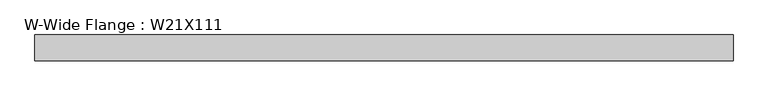
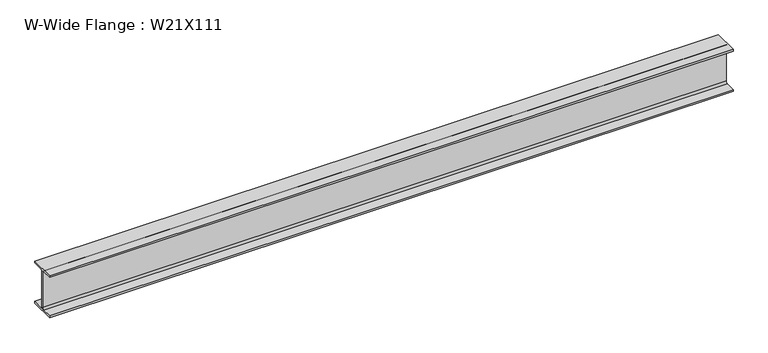
"""IFC4 building model written with IfcOpenShell, lengths in millimetres: beam geometry, W-Wide Flange : W21X111."""

from ifc_helpers import new_model, si_unit, point, frame, frame_2d, origin, place, context, project, spatial, polyline, circle_curve, trimmed, segment, composite_curve, outline, extrude, source, transform, mapped, element, save


def w_wide_flange_w21x111_51b1a384(model_context):
    return source(origin(), model_context, "Body", "SweptSolid", [
        extrude(outline(composite_curve([segment(polyline([(156.21, -250.825), (156.21, -273.05), (-156.21, -273.05), (-156.21, -250.825), (-29.21, -250.825)]), True, "CONTINUOUS"), segment(trimmed(circle_curve(frame_2d((-29.21, -228.6)), 22.225), [point((-29.21, -250.825))], [point((-6.985, -228.6))], True, "CARTESIAN"), True, "CONTINUOUS"), segment(polyline([(-6.985, -228.6), (-6.985, 228.6)]), True, "CONTINUOUS"), segment(trimmed(circle_curve(frame_2d((-29.21, 228.6)), 22.225), [point((-6.985, 228.6))], [point((-29.21, 250.825))], True, "CARTESIAN"), True, "CONTINUOUS"), segment(polyline([(-29.21, 250.825), (-156.21, 250.825), (-156.21, 273.05), (156.21, 273.05), (156.21, 250.825), (29.21, 250.825)]), True, "CONTINUOUS"), segment(trimmed(circle_curve(frame_2d((29.21, 228.6)), 22.225), [point((29.21, 250.825))], [point((6.985, 228.6))], True, "CARTESIAN"), True, "CONTINUOUS"), segment(polyline([(6.985, 228.6), (6.985, -228.6)]), True, "CONTINUOUS"), segment(trimmed(circle_curve(frame_2d((29.21, -228.6)), 22.225), [point((6.985, -228.6))], [point((29.21, -250.825))], True, "CARTESIAN"), True, "CONTINUOUS"), segment(polyline([(29.21, -250.825), (156.21, -250.825)]), True, "CONTINUOUS")], self_intersect=False)), frame((-4220.21, 0.0, 0.0), z_axis=(1.0, 0.0, 0.0), x_axis=(0.0, 1.0, 0.0)), (0.0, 0.0, 1.0), 8440.42),
    ])


if __name__ == "__main__":
    model = new_model("IFC4")
    model_context = context("Model", 3, world=origin())
    ifc_project = project(units=[si_unit("LENGTHUNIT", "METRE", prefix="MILLI")], contexts=[model_context])
    site = spatial("IfcSite", under=ifc_project)
    building = spatial("IfcBuilding", under=site)
    placement = place(None, origin())
    w_wide_flange_w21x111_shape = w_wide_flange_w21x111_51b1a384(model_context)
    element("IfcBeam", 1, ObjectType="W-Wide Flange : W21X111", at=placement, inside=building, context=model_context, shape_type="MappedRepresentation", body=[
        mapped(w_wide_flange_w21x111_shape, transform((0.0, 0.0, 0.0), x_axis=(1.0, 0.0, 0.0), y_axis=(0.0, 1.0, 0.0), z_axis=(0.0, 0.0, 1.0))),
    ])
    save(model, "model.ifc")

# Revit data of these elements
# Type "W-Wide Flange : W21X111"
#   Assembly Code = "B10"
#   W = 111
#   Start Extension Calculation [instance default] = 10' - 0"
#   Start Extension [instance default] = -0' - 0 1/2"
#   End Extension Calculation [instance default] = 10' - 0"
#   End Extension [instance default] = -0' - 0 1/2"
#   Length [instance default] = 5' - 0"
#   bf = 1' - 0.3"
#   d = 1' - 9 1/2"
#   k = 0' - 1 3/4"
#   k2 = 0' - 0 7/8"
#   tf = 0' - 0 7/8"
#   tw = 0' - 0.55"
#   A = 0.227083 SF
#   Beam Material [instance default] = Metal - Steel - ASTM A992
# Element 1 (IfcBeam, "W-Wide Flange : W21X111")
#   Materials on its faces: "Metal - Steel - ASTM A992"
# Materials
#   "Metal - Steel - ASTM A992": class "Metal", colour RGB 128 0 0, transparency 0
